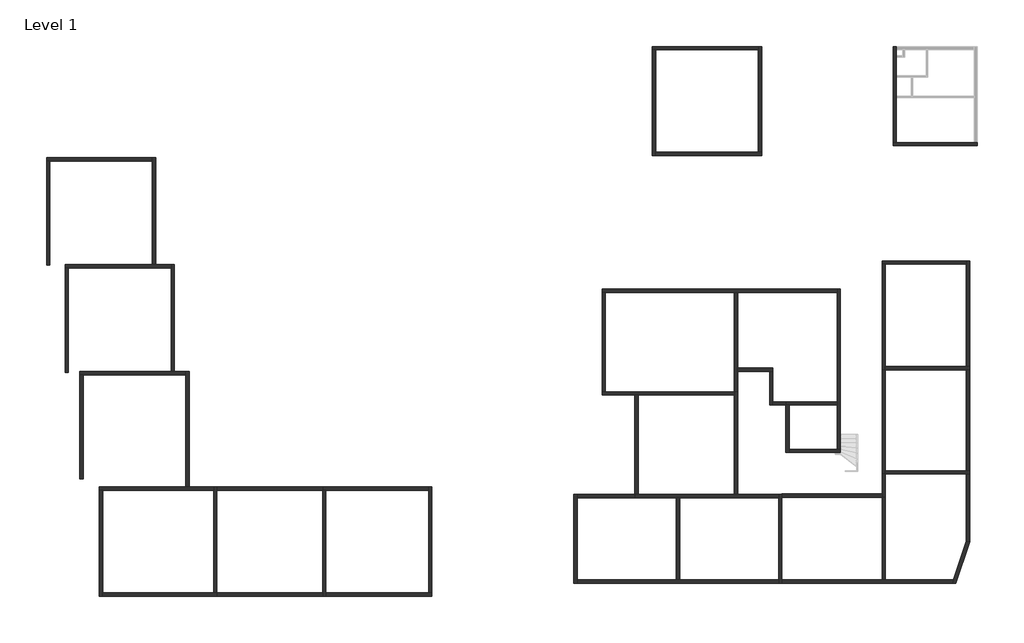
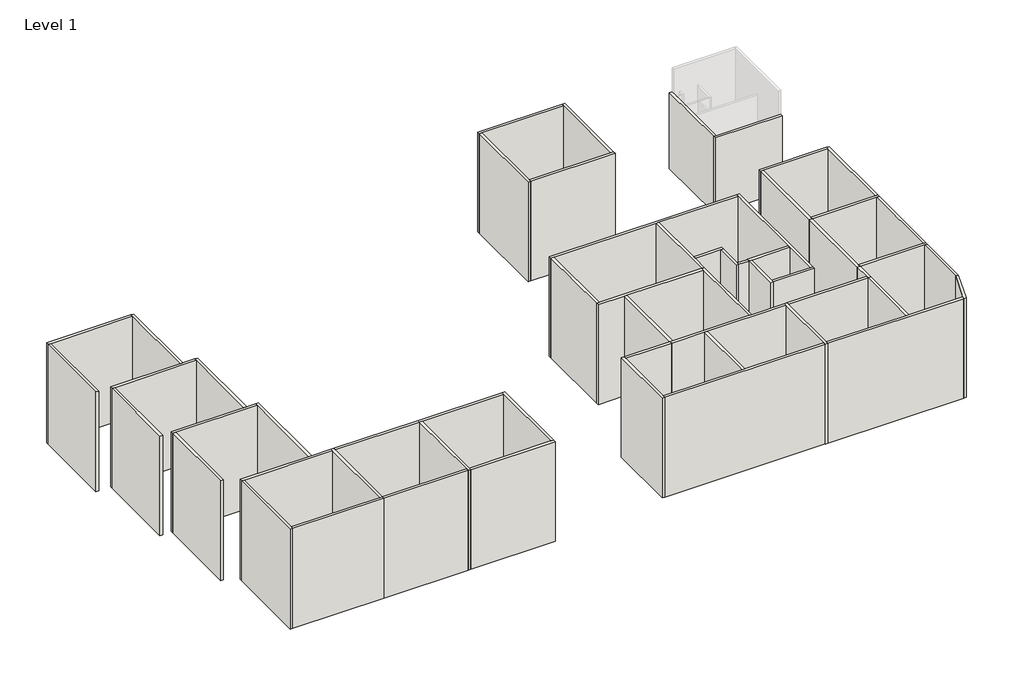
# One storey, part 1 of 2: 57 walls.
"""IFC4 building model written with IfcOpenShell, lengths in millimetres."""

from ifc_helpers import new_model, si_unit, origin, origin_with_axes, place, context, project, spatial, polyline, outline, extrude, faceted_brep, element, save

model = new_model("IFC4")

# Units and contexts
model_context = context("Model", 3, world=origin())
ifc_project = project(units=[si_unit("LENGTHUNIT", "METRE", prefix="MILLI")], contexts=[model_context])

# Site, building, storey
site = spatial("IfcSite", under=ifc_project)
building = spatial("IfcBuilding", under=site)
storey = spatial("IfcBuildingStorey", under=building, Name="Level 1", Elevation=0.0)

# Walls
placement = place(None, origin())
element("IfcWall", 1, ObjectType="Generic - 200mm", at=placement, inside=storey, context=model_context, shape_type="Brep", body=[
    faceted_brep([(30734.9948132, 14981.1915553, 0.0), (30534.9948132, 14981.1915553, 0.0), (25834.9948132, 14981.1915553, 0.0), (25634.9948132, 14981.1915553, 0.0), (25634.9948132, 14981.1915553, 6096.0), (25834.9948132, 14981.1915553, 6096.0), (30734.9948132, 14981.1915553, 6096.0), (30734.9948132, 14781.1915553, 0.0), (30734.9948132, 14781.1915553, 6096.0), (25634.9948132, 14781.1915553, 6096.0), (25634.9948132, 14781.1915553, 0.0)], [[[0, 1, 2, 3, 4, 5, 6]], [[7, 8, 9, 10]], [[3, 2, 1, 0, 7, 10]], [[6, 5, 4, 9, 8]], [[4, 3, 10, 9]], [[0, 6, 8, 7]]]),
])
element("IfcWall", 2, ObjectType="Generic - 200mm", at=placement, inside=storey, context=model_context, shape_type="Brep", body=[
    faceted_brep([(25834.9948132, 14981.1915553, 0.0), (25834.9948132, 17681.1915553, 0.0), (25834.9948132, 17781.1915553, 0.0), (25834.9948132, 18919.7859842, 0.0), (25834.9948132, 19019.7859842, 0.0), (25834.9948132, 20119.7859842, 0.0), (25834.9948132, 20219.7859842, 0.0), (25834.9948132, 20581.1915553, 0.0), (25834.9948132, 20781.1915553, 0.0), (25834.9948132, 20781.1915553, 6096.0), (25834.9948132, 20219.7859842, 6096.0), (25834.9948132, 20119.7859842, 6096.0), (25834.9948132, 19019.7859842, 6096.0), (25834.9948132, 18919.7859842, 6096.0), (25834.9948132, 17781.1915553, 6096.0), (25834.9948132, 17681.1915553, 6096.0), (25834.9948132, 14981.1915553, 6096.0), (25634.9948132, 14981.1915553, 0.0), (25634.9948132, 14981.1915553, 6096.0), (25634.9948132, 20781.1915553, 6096.0), (25634.9948132, 20781.1915553, 0.0)], [[[0, 1, 2, 3, 4, 5, 6, 7, 8, 9, 10, 11, 12, 13, 14, 15, 16]], [[17, 18, 19, 20]], [[8, 7, 6, 5, 4, 3, 2, 1, 0, 17, 20]], [[16, 15, 14, 13, 12, 11, 10, 9, 19, 18]], [[0, 16, 18, 17]], [[9, 8, 20, 19]]]),
])
element("IfcWall", 3, ObjectType="Generic - 200mm", at=placement, inside=storey, context=model_context, shape_type="Brep", body=[
    faceted_brep([(11094.267829, 20581.1915553, 0.0), (11294.267829, 20581.1915553, 0.0), (17494.267829, 20581.1915553, 0.0), (17494.267829, 20581.1915553, 8000.0), (11294.267829, 20581.1915553, 8000.0), (11094.267829, 20581.1915553, 8000.0), (11094.267829, 20781.1915553, 0.0), (11094.267829, 20781.1915553, 8000.0), (17494.267829, 20781.1915553, 8000.0), (17494.267829, 20781.1915553, 0.0)], [[[0, 1, 2, 3, 4, 5]], [[6, 7, 8, 9]], [[2, 1, 0, 6, 9]], [[5, 4, 3, 8, 7]], [[0, 5, 7, 6]], [[3, 2, 9, 8]]]),
])
element("IfcWall", 4, ObjectType="Generic - 200mm", at=placement, inside=storey, context=model_context, shape_type="Brep", body=[
    faceted_brep([(11294.267829, 14181.1915553, 0.0), (11294.267829, 14381.1915553, 0.0), (11294.267829, 20581.1915553, 0.0), (11294.267829, 20581.1915553, 8000.0), (11294.267829, 14381.1915553, 8000.0), (11294.267829, 14181.1915553, 8000.0), (11094.267829, 14181.1915553, 0.0), (11094.267829, 14181.1915553, 8000.0), (11094.267829, 20581.1915553, 8000.0), (11094.267829, 20581.1915553, 0.0)], [[[0, 1, 2, 3, 4, 5]], [[6, 7, 8, 9]], [[2, 1, 0, 6, 9]], [[5, 4, 3, 8, 7]], [[0, 5, 7, 6]], [[3, 2, 9, 8]]]),
])
element("IfcWall", 5, ObjectType="Generic - 200mm", at=placement, inside=storey, context=model_context, shape_type="Brep", body=[
    faceted_brep([(17694.267829, 14381.1915553, 0.0), (17494.267829, 14381.1915553, 0.0), (11294.267829, 14381.1915553, 0.0), (11294.267829, 14381.1915553, 8000.0), (17494.267829, 14381.1915553, 8000.0), (17694.267829, 14381.1915553, 8000.0), (17694.267829, 14181.1915553, 0.0), (17694.267829, 14181.1915553, 8000.0), (11294.267829, 14181.1915553, 8000.0), (11294.267829, 14181.1915553, 0.0)], [[[0, 1, 2, 3, 4, 5]], [[6, 7, 8, 9]], [[2, 1, 0, 6, 9]], [[5, 4, 3, 8, 7]], [[0, 5, 7, 6]], [[3, 2, 9, 8]]]),
])
element("IfcWall", 6, ObjectType="Generic - 200mm", at=placement, inside=storey, context=model_context, shape_type="Brep", body=[
    faceted_brep([(17494.267829, 20781.1915553, 0.0), (17494.267829, 20581.1915553, 0.0), (17494.267829, 14381.1915553, 0.0), (17494.267829, 14381.1915553, 8000.0), (17494.267829, 20581.1915553, 8000.0), (17494.267829, 20781.1915553, 8000.0), (17694.267829, 20781.1915553, 0.0), (17694.267829, 20781.1915553, 8000.0), (17694.267829, 14381.1915553, 8000.0), (17694.267829, 14381.1915553, 0.0)], [[[0, 1, 2, 3, 4, 5]], [[6, 7, 8, 9]], [[2, 1, 0, 6, 9]], [[5, 4, 3, 8, 7]], [[0, 5, 7, 6]], [[3, 2, 9, 8]]]),
])
element("IfcWall", 7, ObjectType="Generic - 200mm", at=placement, inside=storey, context=model_context, shape_type="Brep", body=[
    faceted_brep([(10039.836337, -6505.0098119, 0.0), (12539.836337, -6505.0098119, 0.0), (12739.836337, -6505.0098119, 0.0), (18719.836337, -6505.0098119, 0.0), (18719.836337, -6505.0098119, 8000.0), (12739.836337, -6505.0098119, 8000.0), (12539.836337, -6505.0098119, 8000.0), (10039.836337, -6505.0098119, 8000.0), (10039.836337, -6305.0098119, 0.0), (10039.836337, -6305.0098119, 8000.0), (10239.836337, -6305.0098119, 8000.0), (16039.836337, -6305.0098119, 8000.0), (16239.836337, -6305.0098119, 8000.0), (18719.836337, -6305.0098119, 8000.0), (18719.836337, -6305.0098119, 0.0), (16239.836337, -6305.0098119, 0.0), (16039.836337, -6305.0098119, 0.0), (10239.836337, -6305.0098119, 0.0)], [[[0, 1, 2, 3, 4, 5, 6, 7]], [[8, 9, 10, 11, 12, 13, 14, 15, 16, 17]], [[3, 2, 1, 0, 8, 17, 16, 15, 14]], [[7, 6, 5, 4, 13, 12, 11, 10, 9]], [[4, 3, 14, 13]], [[0, 7, 9, 8]]]),
])
element("IfcWall", 8, ObjectType="Generic - 200mm", at=placement, inside=storey, context=model_context, shape_type="Brep", body=[
    faceted_brep([(6549.836337, -11668.490171, 0.0), (6549.836337, -11468.490171, 0.0), (6549.836337, -6505.0098119, 0.0), (6549.836337, -6305.0098119, 0.0), (6549.836337, -6305.0098119, 8000.0), (6549.836337, -6505.0098119, 8000.0), (6549.836337, -11468.490171, 8000.0), (6549.836337, -11668.490171, 8000.0), (6349.836337, -11668.490171, 0.0), (6349.836337, -11668.490171, 8000.0), (6349.836337, -6305.0098119, 8000.0), (6349.836337, -6305.0098119, 0.0)], [[[0, 1, 2, 3, 4, 5, 6, 7]], [[8, 9, 10, 11]], [[3, 2, 1, 0, 8, 11]], [[7, 6, 5, 4, 10, 9]], [[0, 7, 9, 8]], [[4, 3, 11, 10]]]),
])
element("IfcWall", 9, ObjectType="Generic - 200mm", at=placement, inside=storey, context=model_context, shape_type="Brep", body=[
    faceted_brep([(18719.836337, -11468.490171, 0.0), (12739.836337, -11468.490171, 0.0), (12539.836337, -11468.490171, 0.0), (6549.836337, -11468.490171, 0.0), (6549.836337, -11468.490171, 8000.0), (12539.836337, -11468.490171, 8000.0), (12739.836337, -11468.490171, 8000.0), (18719.836337, -11468.490171, 8000.0), (18719.836337, -11668.490171, 0.0), (18719.836337, -11668.490171, 8000.0), (6549.836337, -11668.490171, 8000.0), (6549.836337, -11668.490171, 0.0)], [[[0, 1, 2, 3, 4, 5, 6, 7]], [[8, 9, 10, 11]], [[3, 2, 1, 0, 8, 11]], [[7, 6, 5, 4, 10, 9]], [[4, 3, 11, 10]], [[0, 7, 9, 8]]]),
])
element("IfcWall", 10, ObjectType="Generic - 200mm", at=placement, inside=storey, context=model_context, shape_type="Brep", body=[
    faceted_brep([(24968.3425199, 7619.475628, 0.0), (25168.3425199, 7619.475628, 0.0), (30068.3425199, 7619.475628, 0.0), (30068.3425199, 7619.475628, 8000.0), (25168.3425199, 7619.475628, 8000.0), (24968.3425199, 7619.475628, 8000.0), (24968.3425199, 7819.475628, 0.0), (24968.3425199, 7819.475628, 8000.0), (30068.3425199, 7819.475628, 8000.0), (30068.3425199, 7819.475628, 0.0)], [[[0, 1, 2, 3, 4, 5]], [[6, 7, 8, 9]], [[2, 1, 0, 6, 9]], [[5, 4, 3, 8, 7]], [[0, 5, 7, 6]], [[3, 2, 9, 8]]]),
])
element("IfcWall", 11, ObjectType="Generic - 200mm", at=placement, inside=storey, context=model_context, shape_type="Brep", body=[
    faceted_brep([(25168.3425199, 1219.475628, 0.0), (25168.3425199, 1419.475628, 0.0), (25168.3425199, 7619.475628, 0.0), (25168.3425199, 7619.475628, 8000.0), (25168.3425199, 1419.475628, 8000.0), (25168.3425199, 1219.475628, 8000.0), (24968.3425199, 1219.475628, 0.0), (24968.3425199, 1219.475628, 8000.0), (24968.3425199, 7619.475628, 8000.0), (24968.3425199, 7619.475628, 0.0), (24968.8612349, 1219.475628, 0.0), (24968.8612349, 1219.475628, 8000.0)], [[[0, 1, 2, 3, 4, 5]], [[6, 7, 8, 9]], [[2, 1, 0, 10, 6, 9]], [[5, 4, 3, 8, 7, 11]], [[0, 5, 11, 7, 6, 10]], [[3, 2, 9, 8]]]),
])
element("IfcWall", 12, ObjectType="Generic - 200mm", at=placement, inside=storey, context=model_context, shape_type="Brep", body=[
    faceted_brep([(30268.3425199, 1419.475628, 0.0), (30068.3425199, 1419.475628, 0.0), (25168.3425199, 1419.475628, 0.0), (25168.3425199, 1419.475628, 8000.0), (30068.3425199, 1419.475628, 8000.0), (30268.3425199, 1419.475628, 8000.0), (30268.3425199, 1219.475628, 0.0), (30268.3425199, 1219.475628, 8000.0), (30068.8612349, 1219.475628, 8000.0), (25168.8612349, 1219.475628, 8000.0), (25168.3425199, 1219.475628, 8000.0), (25168.3425199, 1219.475628, 0.0), (25168.8612349, 1219.475628, 0.0), (30068.8612349, 1219.475628, 0.0)], [[[0, 1, 2, 3, 4, 5]], [[6, 7, 8, 9, 10, 11, 12, 13]], [[2, 1, 0, 6, 13, 12, 11]], [[5, 4, 3, 10, 9, 8, 7]], [[0, 5, 7, 6]], [[3, 2, 11, 10]]]),
])
element("IfcWall", 13, ObjectType="Generic - 200mm", at=placement, inside=storey, context=model_context, shape_type="Brep", body=[
    faceted_brep([(30068.3425199, 7819.475628, 0.0), (30068.3425199, 7619.475628, 0.0), (30068.3425199, 1419.475628, 0.0), (30068.3425199, 1419.475628, 8000.0), (30068.3425199, 7619.475628, 8000.0), (30068.3425199, 7819.475628, 8000.0), (30268.3425199, 7819.475628, 0.0), (30268.3425199, 7819.475628, 8000.0), (30268.3425199, 1419.475628, 8000.0), (30268.3425199, 1419.475628, 0.0)], [[[0, 1, 2, 3, 4, 5]], [[6, 7, 8, 9]], [[2, 1, 0, 6, 9]], [[5, 4, 3, 8, 7]], [[0, 5, 7, 6]], [[3, 2, 9, 8]]]),
])
element("IfcWall", 14, ObjectType="Generic - 200mm", at=placement, inside=storey, context=model_context, shape_type="Brep", body=[
    faceted_brep([(25168.8612349, -5076.2808257, 0.0), (25168.8612349, -4876.2808257, 0.0), (25168.8612349, 1219.475628, 0.0), (25168.8612349, 1219.475628, 8000.0), (25168.8612349, -4876.2808257, 8000.0), (25168.8612349, -5076.2808257, 8000.0), (24968.8612349, -5076.2808257, 0.0), (24968.8612349, -5076.2808257, 8000.0), (24968.8612349, 1219.475628, 8000.0), (24968.8612349, 1219.475628, 0.0), (25168.3425199, 1219.475628, 0.0), (25168.3425199, 1219.475628, 8000.0)], [[[0, 1, 2, 3, 4, 5]], [[6, 7, 8, 9]], [[2, 1, 0, 6, 9, 10]], [[5, 4, 3, 11, 8, 7]], [[0, 5, 7, 6]], [[3, 2, 10, 9, 8, 11]]]),
])
element("IfcWall", 15, ObjectType="Generic - 200mm", at=placement, inside=storey, context=model_context, shape_type="Brep", body=[
    faceted_brep([(30268.8612349, -4876.2808257, 0.0), (30068.8612349, -4876.2808257, 0.0), (25168.8612349, -4876.2808257, 0.0), (25168.8612349, -4876.2808257, 8000.0), (30068.8612349, -4876.2808257, 8000.0), (30268.8612349, -4876.2808257, 8000.0), (30268.8612349, -5076.2808257, 0.0), (30268.8612349, -5076.2808257, 8000.0), (30069.3799498, -5076.2808257, 8000.0), (25168.8612349, -5076.2808257, 8000.0), (25168.8612349, -5076.2808257, 0.0), (30069.3799498, -5076.2808257, 0.0)], [[[0, 1, 2, 3, 4, 5]], [[6, 7, 8, 9, 10, 11]], [[2, 1, 0, 6, 11, 10]], [[5, 4, 3, 9, 8, 7]], [[0, 5, 7, 6]], [[3, 2, 10, 9]]]),
])
element("IfcWall", 16, ObjectType="Generic - 200mm", at=placement, inside=storey, context=model_context, shape_type="Brep", body=[
    faceted_brep([(30068.8612349, 1219.475628, 0.0), (30068.8612349, -4876.2808257, 0.0), (30068.8612349, -4876.2808257, 8000.0), (30068.8612349, 1219.475628, 8000.0), (30268.8612349, 1219.475628, 0.0), (30268.8612349, 1219.475628, 8000.0), (30268.8612349, -4876.2808257, 8000.0), (30268.8612349, -4876.2808257, 0.0), (30268.3425199, 1219.475628, 0.0), (30268.3425199, 1219.475628, 8000.0)], [[[0, 1, 2, 3]], [[4, 5, 6, 7]], [[1, 0, 8, 4, 7]], [[3, 2, 6, 5, 9]], [[2, 1, 7, 6]], [[0, 3, 9, 5, 4, 8]]]),
])
element("IfcWall", 17, ObjectType="Generic - 200mm", at=placement, inside=storey, context=model_context, shape_type="Brep", body=[
    faceted_brep([(30069.3799498, -5076.2808257, 0.0), (30069.3799498, -9143.0251929, 0.0), (30069.3799498, -9143.0251929, 8000.0), (30069.3799498, -5076.2808257, 8000.0), (30269.3799498, -5076.2808257, 0.0), (30269.3799498, -5076.2808257, 8000.0), (30269.3799498, -9175.863443, 8000.0), (30269.3799498, -9175.863443, 0.0), (30268.8612349, -5076.2808257, 0.0), (30268.8612349, -5076.2808257, 8000.0)], [[[0, 1, 2, 3]], [[4, 5, 6, 7]], [[1, 0, 8, 4, 7]], [[3, 2, 6, 5, 9]], [[0, 3, 9, 5, 4, 8]], [[2, 1, 7, 6]]]),
])
element("IfcWall", 18, ObjectType="Generic - 200mm", at=placement, inside=storey, context=model_context, shape_type="Brep", body=[
    faceted_brep([(19150.6041014, -900.524372, 0.0), (19350.6041014, -900.524372, 0.0), (22249.836337, -900.524372, 0.0), (22249.836337, -900.524372, 8000.0), (19350.6041014, -900.524372, 8000.0), (19150.6041014, -900.524372, 8000.0), (19150.6041014, -700.524372, 0.0), (19150.6041014, -700.524372, 8000.0), (22249.836337, -700.524372, 8000.0), (22249.836337, -700.524372, 0.0)], [[[0, 1, 2, 3, 4, 5]], [[6, 7, 8, 9]], [[2, 1, 0, 6, 9]], [[5, 4, 3, 8, 7]], [[0, 5, 7, 6]], [[3, 2, 9, 8]]]),
])
element("IfcWall", 19, ObjectType="Generic - 200mm", at=placement, inside=storey, context=model_context, shape_type="Brep", body=[
    faceted_brep([(19350.6041014, -3776.2808257, 0.0), (19350.6041014, -3576.2808257, 0.0), (19350.6041014, -900.524372, 0.0), (19350.6041014, -900.524372, 8000.0), (19350.6041014, -3576.2808257, 8000.0), (19350.6041014, -3776.2808257, 8000.0), (19150.6041014, -3776.2808257, 0.0), (19150.6041014, -3776.2808257, 8000.0), (19150.6041014, -900.524372, 8000.0), (19150.6041014, -900.524372, 0.0)], [[[0, 1, 2, 3, 4, 5]], [[6, 7, 8, 9]], [[2, 1, 0, 6, 9]], [[5, 4, 3, 8, 7]], [[0, 5, 7, 6]], [[3, 2, 9, 8]]]),
])
element("IfcWall", 20, ObjectType="Generic - 200mm", at=placement, inside=storey, context=model_context, shape_type="Brep", body=[
    faceted_brep([(22449.836337, -3576.2808257, 0.0), (22249.836337, -3576.2808257, 0.0), (19350.6041014, -3576.2808257, 0.0), (19350.6041014, -3576.2808257, 8000.0), (22249.836337, -3576.2808257, 8000.0), (22449.836337, -3576.2808257, 8000.0), (22449.836337, -3776.2808257, 0.0), (22449.836337, -3776.2808257, 8000.0), (19350.6041014, -3776.2808257, 8000.0), (19350.6041014, -3776.2808257, 0.0)], [[[0, 1, 2, 3, 4, 5]], [[6, 7, 8, 9]], [[2, 1, 0, 6, 9]], [[5, 4, 3, 8, 7]], [[3, 2, 9, 8]], [[0, 5, 7, 6]]]),
])
element("IfcWall", 21, ObjectType="Generic - 200mm", at=placement, inside=storey, context=model_context, shape_type="Brep", body=[
    faceted_brep([(18919.836337, -11676.6907835, 0.0), (18919.836337, -11476.6907835, 0.0), (18919.836337, -6476.2808257, 0.0), (18919.836337, -6305.0098119, 0.0), (18919.836337, -6305.0098119, 8000.0), (18919.836337, -6476.2808257, 8000.0), (18919.836337, -11476.6907835, 8000.0), (18919.836337, -11676.6907835, 8000.0), (18719.836337, -11676.6907835, 0.0), (18719.836337, -11676.6907835, 8000.0), (18719.836337, -11668.490171, 8000.0), (18719.836337, -11468.490171, 8000.0), (18719.836337, -6505.0098119, 8000.0), (18719.836337, -6305.0098119, 8000.0), (18719.836337, -6305.0098119, 0.0), (18719.836337, -6505.0098119, 0.0), (18719.836337, -11468.490171, 0.0), (18719.836337, -11668.490171, 0.0)], [[[0, 1, 2, 3, 4, 5, 6, 7]], [[8, 9, 10, 11, 12, 13, 14, 15, 16, 17]], [[3, 2, 1, 0, 8, 17, 16, 15, 14]], [[7, 6, 5, 4, 13, 12, 11, 10, 9]], [[0, 7, 9, 8]], [[4, 3, 14, 13]]]),
])
element("IfcWall", 22, ObjectType="Generic - 200mm", at=placement, inside=storey, context=model_context, shape_type="Brep", body=[
    faceted_brep([(29281.8131798, -11476.6907835, 0.0), (25168.8612349, -11476.6907835, 0.0), (24968.8612349, -11476.6907835, 0.0), (18919.836337, -11476.6907835, 0.0), (18919.836337, -11476.6907835, 8000.0), (24968.8612349, -11476.6907835, 8000.0), (25168.8612349, -11476.6907835, 8000.0), (29281.8131798, -11476.6907835, 8000.0), (29214.3170678, -11676.6907835, 0.0), (29214.3170678, -11676.6907835, 8000.0), (18919.836337, -11676.6907835, 8000.0), (18919.836337, -11676.6907835, 0.0)], [[[0, 1, 2, 3, 4, 5, 6, 7]], [[8, 9, 10, 11]], [[3, 2, 1, 0, 8, 11]], [[7, 6, 5, 4, 10, 9]], [[4, 3, 11, 10]], [[0, 7, 9, 8]]]),
])
element("IfcWall", 23, ObjectType="Generic - 200mm", at=placement, inside=storey, context=model_context, shape_type="Brep", body=[
    faceted_brep([(22449.836337, -3576.2808257, 0.0), (22449.836337, 6101.390757, 0.0), (22449.836337, 6101.390757, 8000.0), (22449.836337, -3576.2808257, 8000.0), (22249.836337, -3576.2808257, 0.0), (22249.836337, -3576.2808257, 8000.0), (22249.836337, -900.524372, 8000.0), (22249.836337, -700.524372, 8000.0), (22249.836337, 5901.390757, 8000.0), (22249.836337, 6101.390757, 8000.0), (22249.836337, 6101.390757, 0.0), (22249.836337, 5901.390757, 0.0), (22249.836337, -700.524372, 0.0), (22249.836337, -900.524372, 0.0)], [[[0, 1, 2, 3]], [[4, 5, 6, 7, 8, 9, 10, 11, 12, 13]], [[1, 0, 4, 13, 12, 11, 10]], [[3, 2, 9, 8, 7, 6, 5]], [[0, 3, 5, 4]], [[2, 1, 10, 9]]]),
])
element("IfcWall", 24, ObjectType="Generic - 200mm", at=placement, inside=storey, context=model_context, shape_type="Brep", body=[
    faceted_brep([(-2430.0032836, -5850.5375199, 0.0), (-2430.0032836, -6050.5375199, 0.0), (-2430.0032836, -12250.5375199, 0.0), (-2430.0032836, -12250.5375199, 8000.0), (-2430.0032836, -6050.5375199, 8000.0), (-2430.0032836, -5850.5375199, 8000.0), (-2230.0032836, -5850.5375199, 0.0), (-2230.0032836, -5850.5375199, 8000.0), (-2230.0032836, -12250.5375199, 8000.0), (-2230.0032836, -12250.5375199, 0.0)], [[[0, 1, 2, 3, 4, 5]], [[6, 7, 8, 9]], [[2, 1, 0, 6, 9]], [[5, 4, 3, 8, 7]], [[0, 5, 7, 6]], [[3, 2, 9, 8]]]),
])
element("IfcWall", 25, ObjectType="Generic - 200mm", at=placement, inside=storey, context=model_context, shape_type="Brep", body=[
    faceted_brep([(-8830.0032836, -6050.5375199, 0.0), (-8630.0032836, -6050.5375199, 0.0), (-2430.0032836, -6050.5375199, 0.0), (-2430.0032836, -6050.5375199, 8000.0), (-8630.0032836, -6050.5375199, 8000.0), (-8830.0032836, -6050.5375199, 8000.0), (-8830.0032836, -5850.5375199, 0.0), (-8830.0032836, -5850.5375199, 8000.0), (-2430.0032836, -5850.5375199, 8000.0), (-2430.0032836, -5850.5375199, 0.0), (-8830.0032836, -5851.0562349, 0.0), (-8830.0032836, -5851.0562349, 8000.0)], [[[0, 1, 2, 3, 4, 5]], [[6, 7, 8, 9]], [[2, 1, 0, 10, 6, 9]], [[5, 4, 3, 8, 7, 11]], [[0, 5, 11, 7, 6, 10]], [[3, 2, 9, 8]]]),
])
element("IfcWall", 26, ObjectType="Generic - 200mm", at=placement, inside=storey, context=model_context, shape_type="Brep", body=[
    faceted_brep([(-8630.0032836, -12450.5375199, 0.0), (-8630.0032836, -12250.5375199, 0.0), (-8630.0032836, -6050.5375199, 0.0), (-8630.0032836, -6050.5375199, 8000.0), (-8630.0032836, -12250.5375199, 8000.0), (-8630.0032836, -12450.5375199, 8000.0), (-8830.0032836, -12450.5375199, 0.0), (-8830.0032836, -12450.5375199, 8000.0), (-8830.0032836, -12251.0562349, 8000.0), (-8830.0032836, -6051.0562349, 8000.0), (-8830.0032836, -6050.5375199, 8000.0), (-8830.0032836, -6050.5375199, 0.0), (-8830.0032836, -6051.0562349, 0.0), (-8830.0032836, -12251.0562349, 0.0)], [[[0, 1, 2, 3, 4, 5]], [[6, 7, 8, 9, 10, 11, 12, 13]], [[2, 1, 0, 6, 13, 12, 11]], [[5, 4, 3, 10, 9, 8, 7]], [[0, 5, 7, 6]], [[3, 2, 11, 10]]]),
])
element("IfcWall", 27, ObjectType="Generic - 200mm", at=placement, inside=storey, context=model_context, shape_type="Brep", body=[
    faceted_brep([(-2230.0032836, -12250.5375199, 0.0), (-2430.0032836, -12250.5375199, 0.0), (-8630.0032836, -12250.5375199, 0.0), (-8630.0032836, -12250.5375199, 8000.0), (-2430.0032836, -12250.5375199, 8000.0), (-2230.0032836, -12250.5375199, 8000.0), (-2230.0032836, -12450.5375199, 0.0), (-2230.0032836, -12450.5375199, 8000.0), (-8630.0032836, -12450.5375199, 8000.0), (-8630.0032836, -12450.5375199, 0.0)], [[[0, 1, 2, 3, 4, 5]], [[6, 7, 8, 9]], [[2, 1, 0, 6, 9]], [[5, 4, 3, 8, 7]], [[0, 5, 7, 6]], [[3, 2, 9, 8]]]),
])
element("IfcWall", 28, ObjectType="Generic - 200mm", at=placement, inside=storey, context=model_context, shape_type="Brep", body=[
    faceted_brep([(-15225.7597372, -6051.0562349, 0.0), (-8830.0032836, -6051.0562349, 0.0), (-8830.0032836, -6051.0562349, 8000.0), (-15225.7597372, -6051.0562349, 8000.0), (-15225.7597372, -5851.0562349, 0.0), (-15225.7597372, -5851.0562349, 8000.0), (-8830.0032836, -5851.0562349, 8000.0), (-8830.0032836, -5851.0562349, 0.0), (-8830.0032836, -6050.5375199, 0.0), (-8830.0032836, -6050.5375199, 8000.0)], [[[0, 1, 2, 3]], [[4, 5, 6, 7]], [[1, 0, 4, 7, 8]], [[3, 2, 9, 6, 5]], [[2, 1, 8, 7, 6, 9]], [[0, 3, 5, 4]]]),
])
element("IfcWall", 29, ObjectType="Generic - 200mm", at=placement, inside=storey, context=model_context, shape_type="Brep", body=[
    faceted_brep([(-8830.0032836, -12251.0562349, 0.0), (-15225.7597372, -12251.0562349, 0.0), (-15225.7597372, -12251.0562349, 8000.0), (-8830.0032836, -12251.0562349, 8000.0), (-8830.0032836, -12451.0562349, 0.0), (-8830.0032836, -12451.0562349, 8000.0), (-15225.7597372, -12451.0562349, 8000.0), (-15225.7597372, -12451.0562349, 0.0), (-8830.0032836, -12450.5375199, 0.0), (-8830.0032836, -12450.5375199, 8000.0)], [[[0, 1, 2, 3]], [[4, 5, 6, 7]], [[1, 0, 8, 4, 7]], [[3, 2, 6, 5, 9]], [[0, 3, 9, 5, 4, 8]], [[2, 1, 7, 6]]]),
])
element("IfcWall", 30, ObjectType="Generic - 200mm", at=placement, inside=storey, context=model_context, shape_type="Brep", body=[
    faceted_brep([(-25515.2414934, 13854.6128579, 0.0), (-25315.2414934, 13854.6128579, 0.0), (-19115.2414934, 13854.6128579, 0.0), (-19115.2414934, 13854.6128579, 8000.0), (-25315.2414934, 13854.6128579, 8000.0), (-25515.2414934, 13854.6128579, 8000.0), (-25515.2414934, 14054.6128579, 0.0), (-25515.2414934, 14054.6128579, 8000.0), (-19115.2414934, 14054.6128579, 8000.0), (-19115.2414934, 14054.6128579, 0.0)], [[[0, 1, 2, 3, 4, 5]], [[6, 7, 8, 9]], [[2, 1, 0, 6, 9]], [[5, 4, 3, 8, 7]], [[0, 5, 7, 6]], [[3, 2, 9, 8]]]),
])
element("IfcWall", 31, ObjectType="Generic - 200mm", at=placement, inside=storey, context=model_context, shape_type="SweptSolid", body=[
    extrude(outline(polyline([(-25315.2414934, 13854.6128579), (-25315.2414934, 7554.6128579), (-25515.2414934, 7554.6128579), (-25515.2414934, 13854.6128579), (-25315.2414934, 13854.6128579)])), origin_with_axes(), (0.0, 0.0, 1.0), 8000.0),
])
element("IfcWall", 32, ObjectType="Generic - 200mm", at=placement, inside=storey, context=model_context, shape_type="Brep", body=[
    faceted_brep([(-19115.2414934, 14054.6128579, 0.0), (-19115.2414934, 13854.6128579, 0.0), (-19115.2414934, 7585.232767, 0.0), (-19115.2414934, 7585.232767, 8000.0), (-19115.2414934, 13854.6128579, 8000.0), (-19115.2414934, 14054.6128579, 8000.0), (-18915.2414934, 14054.6128579, 0.0), (-18915.2414934, 14054.6128579, 8000.0), (-18915.2414934, 7585.232767, 8000.0), (-18915.2414934, 7585.232767, 0.0)], [[[0, 1, 2, 3, 4, 5]], [[6, 7, 8, 9]], [[2, 1, 0, 6, 9]], [[5, 4, 3, 8, 7]], [[0, 5, 7, 6]], [[3, 2, 9, 8]]]),
])
element("IfcWall", 33, ObjectType="Generic - 200mm", at=placement, inside=storey, context=model_context, shape_type="Brep", body=[
    faceted_brep([(-24394.8529907, 7385.232767, 0.0), (-24194.8529907, 7385.232767, 0.0), (-17994.8529907, 7385.232767, 0.0), (-17994.8529907, 7385.232767, 8000.0), (-24194.8529907, 7385.232767, 8000.0), (-24394.8529907, 7385.232767, 8000.0), (-24394.8529907, 7585.232767, 0.0), (-24394.8529907, 7585.232767, 8000.0), (-19115.2414934, 7585.232767, 8000.0), (-18915.2414934, 7585.232767, 8000.0), (-17994.8529907, 7585.232767, 8000.0), (-17994.8529907, 7585.232767, 0.0), (-18915.2414934, 7585.232767, 0.0), (-19115.2414934, 7585.232767, 0.0)], [[[0, 1, 2, 3, 4, 5]], [[6, 7, 8, 9, 10, 11, 12, 13]], [[2, 1, 0, 6, 13, 12, 11]], [[5, 4, 3, 10, 9, 8, 7]], [[0, 5, 7, 6]], [[3, 2, 11, 10]]]),
])
element("IfcWall", 34, ObjectType="Generic - 200mm", at=placement, inside=storey, context=model_context, shape_type="SweptSolid", body=[
    extrude(outline(polyline([(-24194.8529907, 7385.232767), (-24194.8529907, 1085.232767), (-24394.8529907, 1085.232767), (-24394.8529907, 7385.232767), (-24194.8529907, 7385.232767)])), origin_with_axes(), (0.0, 0.0, 1.0), 8000.0),
])
element("IfcWall", 35, ObjectType="Generic - 200mm", at=placement, inside=storey, context=model_context, shape_type="Brep", body=[
    faceted_brep([(-17994.8529907, 7585.232767, 0.0), (-17994.8529907, 7385.232767, 0.0), (-17994.8529907, 1134.2648187, 0.0), (-17994.8529907, 1134.2648187, 8000.0), (-17994.8529907, 7385.232767, 8000.0), (-17994.8529907, 7585.232767, 8000.0), (-17794.8529907, 7585.232767, 0.0), (-17794.8529907, 7585.232767, 8000.0), (-17794.8529907, 1134.2648187, 8000.0), (-17794.8529907, 1134.2648187, 0.0)], [[[0, 1, 2, 3, 4, 5]], [[6, 7, 8, 9]], [[2, 1, 0, 6, 9]], [[5, 4, 3, 8, 7]], [[0, 5, 7, 6]], [[3, 2, 9, 8]]]),
])
element("IfcWall", 36, ObjectType="Generic - 200mm", at=placement, inside=storey, context=model_context, shape_type="Brep", body=[
    faceted_brep([(-23499.9022694, 934.2648187, 0.0), (-23299.9022694, 934.2648187, 0.0), (-17099.9022694, 934.2648187, 0.0), (-17099.9022694, 934.2648187, 8000.0), (-23299.9022694, 934.2648187, 8000.0), (-23499.9022694, 934.2648187, 8000.0), (-23499.9022694, 1134.2648187, 0.0), (-23499.9022694, 1134.2648187, 8000.0), (-17994.8529907, 1134.2648187, 8000.0), (-17794.8529907, 1134.2648187, 8000.0), (-17099.9022694, 1134.2648187, 8000.0), (-17099.9022694, 1134.2648187, 0.0), (-17794.8529907, 1134.2648187, 0.0), (-17994.8529907, 1134.2648187, 0.0)], [[[0, 1, 2, 3, 4, 5]], [[6, 7, 8, 9, 10, 11, 12, 13]], [[2, 1, 0, 6, 13, 12, 11]], [[5, 4, 3, 10, 9, 8, 7]], [[0, 5, 7, 6]], [[3, 2, 11, 10]]]),
])
element("IfcWall", 37, ObjectType="Generic - 200mm", at=placement, inside=storey, context=model_context, shape_type="SweptSolid", body=[
    extrude(outline(polyline([(-23299.9022694, 934.2648187), (-23299.9022694, -5365.7351813), (-23499.9022694, -5365.7351813), (-23499.9022694, 934.2648187), (-23299.9022694, 934.2648187)])), origin_with_axes(), (0.0, 0.0, 1.0), 8000.0),
])
element("IfcWall", 38, ObjectType="Generic - 200mm", at=placement, inside=storey, context=model_context, shape_type="Brep", body=[
    faceted_brep([(-17099.9022694, 1134.2648187, 0.0), (-17099.9022694, 934.2648187, 0.0), (-17099.9022694, -5851.0562349, 0.0), (-17099.9022694, -5851.0562349, 8000.0), (-17099.9022694, 934.2648187, 8000.0), (-17099.9022694, 1134.2648187, 8000.0), (-16899.9022694, 1134.2648187, 0.0), (-16899.9022694, 1134.2648187, 8000.0), (-16899.9022694, -5851.0562349, 8000.0), (-16899.9022694, -5851.0562349, 0.0)], [[[0, 1, 2, 3, 4, 5]], [[6, 7, 8, 9]], [[2, 1, 0, 6, 9]], [[5, 4, 3, 8, 7]], [[0, 5, 7, 6]], [[3, 2, 9, 8]]]),
])
element("IfcWall", 39, ObjectType="Generic - 200mm", at=placement, inside=storey, context=model_context, shape_type="Brep", body=[
    faceted_brep([(-22325.7597372, -6051.0562349, 0.0), (-22125.7597372, -6051.0562349, 0.0), (-15425.7597372, -6051.0562349, 0.0), (-15425.7597372, -6051.0562349, 8000.0), (-22125.7597372, -6051.0562349, 8000.0), (-22325.7597372, -6051.0562349, 8000.0), (-22325.7597372, -5851.0562349, 0.0), (-22325.7597372, -5851.0562349, 8000.0), (-17099.9022694, -5851.0562349, 8000.0), (-16899.9022694, -5851.0562349, 8000.0), (-15425.7597372, -5851.0562349, 8000.0), (-15425.7597372, -5851.0562349, 0.0), (-16899.9022694, -5851.0562349, 0.0), (-17099.9022694, -5851.0562349, 0.0)], [[[0, 1, 2, 3, 4, 5]], [[6, 7, 8, 9, 10, 11, 12, 13]], [[2, 1, 0, 6, 13, 12, 11]], [[5, 4, 3, 10, 9, 8, 7]], [[0, 5, 7, 6]], [[3, 2, 11, 10]]]),
])
element("IfcWall", 40, ObjectType="Generic - 200mm", at=placement, inside=storey, context=model_context, shape_type="Brep", body=[
    faceted_brep([(-22125.7597372, -12451.0562349, 0.0), (-22125.7597372, -12251.0562349, 0.0), (-22125.7597372, -6051.0562349, 0.0), (-22125.7597372, -6051.0562349, 8000.0), (-22125.7597372, -12251.0562349, 8000.0), (-22125.7597372, -12451.0562349, 8000.0), (-22325.7597372, -12451.0562349, 0.0), (-22325.7597372, -12451.0562349, 8000.0), (-22325.7597372, -6051.0562349, 8000.0), (-22325.7597372, -6051.0562349, 0.0)], [[[0, 1, 2, 3, 4, 5]], [[6, 7, 8, 9]], [[2, 1, 0, 6, 9]], [[5, 4, 3, 8, 7]], [[0, 5, 7, 6]], [[3, 2, 9, 8]]]),
])
element("IfcWall", 41, ObjectType="Generic - 200mm", at=placement, inside=storey, context=model_context, shape_type="Brep", body=[
    faceted_brep([(-15225.7597372, -12251.0562349, 0.0), (-15425.7597372, -12251.0562349, 0.0), (-22125.7597372, -12251.0562349, 0.0), (-22125.7597372, -12251.0562349, 8000.0), (-15425.7597372, -12251.0562349, 8000.0), (-15225.7597372, -12251.0562349, 8000.0), (-15225.7597372, -12451.0562349, 0.0), (-15225.7597372, -12451.0562349, 8000.0), (-22125.7597372, -12451.0562349, 8000.0), (-22125.7597372, -12451.0562349, 0.0)], [[[0, 1, 2, 3, 4, 5]], [[6, 7, 8, 9]], [[2, 1, 0, 6, 9]], [[5, 4, 3, 8, 7]], [[0, 5, 7, 6]], [[3, 2, 9, 8]]]),
])
element("IfcWall", 42, ObjectType="Generic - 200mm", at=placement, inside=storey, context=model_context, shape_type="Brep", body=[
    faceted_brep([(-15425.7597372, -5851.0562349, 0.0), (-15425.7597372, -6051.0562349, 0.0), (-15425.7597372, -12251.0562349, 0.0), (-15425.7597372, -12251.0562349, 8000.0), (-15425.7597372, -6051.0562349, 8000.0), (-15425.7597372, -5851.0562349, 8000.0), (-15225.7597372, -5851.0562349, 0.0), (-15225.7597372, -5851.0562349, 8000.0), (-15225.7597372, -6051.0562349, 8000.0), (-15225.7597372, -12251.0562349, 8000.0), (-15225.7597372, -12251.0562349, 0.0), (-15225.7597372, -6051.0562349, 0.0)], [[[0, 1, 2, 3, 4, 5]], [[6, 7, 8, 9, 10, 11]], [[2, 1, 0, 6, 11, 10]], [[5, 4, 3, 9, 8, 7]], [[0, 5, 7, 6]], [[3, 2, 10, 9]]]),
])
element("IfcWall", 43, ObjectType="Generic - 200mm", at=placement, inside=storey, context=model_context, shape_type="Brep", body=[
    faceted_brep([(16039.836337, -98.609243, 0.0), (16039.836337, -298.609243, 0.0), (16039.836337, -6305.0098119, 0.0), (16039.836337, -6305.0098119, 8000.0), (16039.836337, -298.609243, 8000.0), (16039.836337, -98.609243, 8000.0), (16239.836337, -98.609243, 0.0), (16239.836337, -98.609243, 8000.0), (16239.836337, -6305.0098119, 8000.0), (16239.836337, -6305.0098119, 0.0)], [[[0, 1, 2, 3, 4, 5]], [[6, 7, 8, 9]], [[2, 1, 0, 6, 9]], [[5, 4, 3, 8, 7]], [[3, 2, 9, 8]], [[0, 5, 7, 6]]]),
])
element("IfcWall", 44, ObjectType="Generic - 200mm", at=placement, inside=storey, context=model_context, shape_type="Brep", body=[
    faceted_brep([(8048.9259597, -298.609243, 0.0), (10039.836337, -298.609243, 0.0), (10239.836337, -298.609243, 0.0), (16039.836337, -298.609243, 0.0), (16039.836337, -298.609243, 8000.0), (10239.836337, -298.609243, 8000.0), (10039.836337, -298.609243, 8000.0), (8048.9259597, -298.609243, 8000.0), (8048.9259597, -98.609243, 0.0), (8048.9259597, -98.609243, 8000.0), (8248.9259597, -98.609243, 8000.0), (16039.836337, -98.609243, 8000.0), (16039.836337, -98.609243, 0.0), (8248.9259597, -98.609243, 0.0)], [[[0, 1, 2, 3, 4, 5, 6, 7]], [[8, 9, 10, 11, 12, 13]], [[3, 2, 1, 0, 8, 13, 12]], [[7, 6, 5, 4, 11, 10, 9]], [[4, 3, 12, 11]], [[0, 7, 9, 8]]]),
])
element("IfcWall", 45, ObjectType="Generic - 200mm", at=placement, inside=storey, context=model_context, shape_type="Brep", body=[
    faceted_brep([(8048.9259597, 5901.390757, 0.0), (8248.9259597, 5901.390757, 0.0), (16039.836337, 5901.390757, 0.0), (16239.836337, 5901.390757, 0.0), (22249.836337, 5901.390757, 0.0), (22249.836337, 5901.390757, 8000.0), (16239.836337, 5901.390757, 8000.0), (16039.836337, 5901.390757, 8000.0), (8248.9259597, 5901.390757, 8000.0), (8048.9259597, 5901.390757, 8000.0), (8048.9259597, 6101.390757, 0.0), (8048.9259597, 6101.390757, 8000.0), (22249.836337, 6101.390757, 8000.0), (22249.836337, 6101.390757, 0.0)], [[[0, 1, 2, 3, 4, 5, 6, 7, 8, 9]], [[10, 11, 12, 13]], [[4, 3, 2, 1, 0, 10, 13]], [[9, 8, 7, 6, 5, 12, 11]], [[5, 4, 13, 12]], [[0, 9, 11, 10]]]),
])
element("IfcWall", 46, ObjectType="Generic - 200mm", at=placement, inside=storey, context=model_context, shape_type="SweptSolid", body=[
    extrude(outline(polyline([(24968.8612349, -11476.6907835), (24968.8612349, -6476.2808257), (25168.8612349, -6476.2808257), (25168.8612349, -11476.6907835), (24968.8612349, -11476.6907835)])), origin_with_axes(), (0.0, 0.0, 1.0), 8000.0),
])
element("IfcWall", 47, ObjectType="Generic - 200mm", at=placement, inside=storey, context=model_context, shape_type="Brep", body=[
    faceted_brep([(30069.3799498, -9143.0251929, 0.0), (29281.8131798, -11476.6907835, 0.0), (29214.3170678, -11676.6907835, 0.0), (29214.3170678, -11676.6907835, 8000.0), (29281.8131798, -11476.6907835, 8000.0), (30069.3799498, -9143.0251929, 8000.0), (30269.3799498, -9175.863443, 0.0), (30269.3799498, -9175.863443, 8000.0), (29425.3993388, -11676.6907835, 8000.0), (29425.3993388, -11676.6907835, 0.0)], [[[0, 1, 2, 3, 4, 5]], [[6, 7, 8, 9]], [[2, 1, 0, 6, 9]], [[5, 4, 3, 8, 7]], [[0, 5, 7, 6]], [[3, 2, 9, 8]]]),
])
element("IfcWall", 48, ObjectType="Generic - 200mm", at=placement, inside=storey, context=model_context, shape_type="Brep", body=[
    faceted_brep([(24968.8612349, -5076.2808257, 0.0), (24968.8612349, -6276.2808257, 0.0), (24968.8612349, -6476.2808257, 0.0), (24968.8612349, -6476.2808257, 8000.0), (24968.8612349, -6276.2808257, 8000.0), (24968.8612349, -5076.2808257, 8000.0), (25168.8612349, -5076.2808257, 0.0), (25168.8612349, -5076.2808257, 8000.0), (25168.8612349, -6476.2808257, 8000.0), (25168.8612349, -6476.2808257, 0.0)], [[[0, 1, 2, 3, 4, 5]], [[6, 7, 8, 9]], [[2, 1, 0, 6, 9]], [[5, 4, 3, 8, 7]], [[0, 5, 7, 6]], [[3, 2, 9, 8]]]),
])
element("IfcWall", 49, ObjectType="Generic - 200mm", at=placement, inside=storey, context=model_context, shape_type="Brep", body=[
    faceted_brep([(24968.8612349, -6276.2808257, 0.0), (18919.836337, -6276.2808257, 0.0), (18919.836337, -6276.2808257, 8000.0), (24968.8612349, -6276.2808257, 8000.0), (24968.8612349, -6476.2808257, 0.0), (24968.8612349, -6476.2808257, 8000.0), (18919.836337, -6476.2808257, 8000.0), (18919.836337, -6476.2808257, 0.0), (18919.836337, -6305.0098119, 0.0), (18919.836337, -6305.0098119, 8000.0)], [[[0, 1, 2, 3]], [[4, 5, 6, 7]], [[1, 0, 4, 7, 8]], [[3, 2, 9, 6, 5]], [[0, 3, 5, 4]], [[2, 1, 8, 7, 6, 9]]]),
])
element("IfcWall", 50, ObjectType="Generic - 200mm", at=placement, inside=storey, context=model_context, shape_type="SweptSolid", body=[
    extrude(outline(polyline([(12539.836337, -11468.490171), (12539.836337, -6505.0098119), (12739.836337, -6505.0098119), (12739.836337, -11468.490171), (12539.836337, -11468.490171)])), origin_with_axes(), (0.0, 0.0, 1.0), 8000.0),
])
element("IfcWall", 51, ObjectType="Generic - 200mm", at=placement, inside=storey, context=model_context, shape_type="SweptSolid", body=[
    extrude(outline(polyline([(10039.836337, -6305.0098119), (10039.836337, -298.609243), (10239.836337, -298.609243), (10239.836337, -6305.0098119), (10039.836337, -6305.0098119)])), origin_with_axes(), (0.0, 0.0, 1.0), 8000.0),
])
element("IfcWall", 52, ObjectType="Generic - 200mm", at=placement, inside=storey, context=model_context, shape_type="SweptSolid", body=[
    extrude(outline(polyline([(8048.9259597, -98.609243), (8048.9259597, 5901.390757), (8248.9259597, 5901.390757), (8248.9259597, -98.609243), (8048.9259597, -98.609243)])), origin_with_axes(), (0.0, 0.0, 1.0), 8000.0),
])
element("IfcWall", 53, ObjectType="Generic - 200mm", at=placement, inside=storey, context=model_context, shape_type="SweptSolid", body=[
    extrude(outline(polyline([(6549.836337, -6305.0098119), (10039.836337, -6305.0098119), (10039.836337, -6505.0098119), (6549.836337, -6505.0098119), (6549.836337, -6305.0098119)])), origin_with_axes(), (0.0, 0.0, 1.0), 8000.0),
])
element("IfcWall", 54, ObjectType="Generic - 200mm", at=placement, inside=storey, context=model_context, shape_type="Brep", body=[
    faceted_brep([(16239.836337, -98.609243, 0.0), (16239.836337, 1139.475628, 0.0), (16239.836337, 1339.475628, 0.0), (16239.836337, 5901.390757, 0.0), (16239.836337, 5901.390757, 8000.0), (16239.836337, 1339.475628, 8000.0), (16239.836337, 1139.475628, 8000.0), (16239.836337, -98.609243, 8000.0), (16039.836337, -98.609243, 0.0), (16039.836337, -98.609243, 8000.0), (16039.836337, 5901.390757, 8000.0), (16039.836337, 5901.390757, 0.0)], [[[0, 1, 2, 3, 4, 5, 6, 7]], [[8, 9, 10, 11]], [[3, 2, 1, 0, 8, 11]], [[7, 6, 5, 4, 10, 9]], [[0, 7, 9, 8]], [[4, 3, 11, 10]]]),
])
element("IfcWall", 55, ObjectType="Generic - 200mm", at=placement, inside=storey, context=model_context, shape_type="Brep", body=[
    faceted_brep([(16239.836337, 1139.475628, 0.0), (18179.836337, 1139.475628, 0.0), (18379.836337, 1139.475628, 0.0), (18379.836337, 1139.475628, 8000.0), (18179.836337, 1139.475628, 8000.0), (16239.836337, 1139.475628, 8000.0), (16239.836337, 1339.475628, 0.0), (16239.836337, 1339.475628, 8000.0), (18379.836337, 1339.475628, 8000.0), (18379.836337, 1339.475628, 0.0)], [[[0, 1, 2, 3, 4, 5]], [[6, 7, 8, 9]], [[2, 1, 0, 6, 9]], [[5, 4, 3, 8, 7]], [[0, 5, 7, 6]], [[3, 2, 9, 8]]]),
])
element("IfcWall", 56, ObjectType="Generic - 200mm", at=placement, inside=storey, context=model_context, shape_type="Brep", body=[
    faceted_brep([(18179.836337, 1139.475628, 0.0), (18179.836337, -900.524372, 0.0), (18179.836337, -900.524372, 8000.0), (18179.836337, 1139.475628, 8000.0), (18379.836337, 1139.475628, 0.0), (18379.836337, 1139.475628, 8000.0), (18379.836337, -700.524372, 8000.0), (18379.836337, -900.524372, 8000.0), (18379.836337, -900.524372, 0.0), (18379.836337, -700.524372, 0.0)], [[[0, 1, 2, 3]], [[4, 5, 6, 7, 8, 9]], [[1, 0, 4, 9, 8]], [[3, 2, 7, 6, 5]], [[0, 3, 5, 4]], [[2, 1, 8, 7]]]),
])
element("IfcWall", 57, ObjectType="Generic - 200mm", at=placement, inside=storey, context=model_context, shape_type="SweptSolid", body=[
    extrude(outline(polyline([(19139.836337, -900.524372), (18379.836337, -900.524372), (18379.836337, -700.524372), (19139.836337, -700.524372), (19139.836337, -900.524372)])), origin_with_axes(), (0.0, 0.0, 1.0), 8000.0),
])

save(model, "model.ifc")

# Revit data of these elements
# Project information
#   Project Issue Date = "Issue Date"
#   Project Status = "Project Status"
#   Client Name = "Owner"
#   Project Address = "Enter address here"
#   Project Name = "Project Name"
#   Project Number = "0001"
# Type "Generic - 200mm"
#   Layers, outside or top first: 20 cm no material (function 1)
# Elements 1, 2 (IfcWall, "Generic - 200mm")
#   Top Offset = 0 cm
#   Base Offset = 0 cm
#   Unconnected Height = 609.6 cm
#   wall height = 609.6 cm
#   Phase Created = New Construction
#   Base Constraint = Level 1
#   Materials on its faces: "Default Wall"
# Elements 3, 4, 5, 6, 7, 8, 9, 10, 11, 12, 13, 14, 15, 16, 17, 18, 19, 20, 21, 22, 23, 24, 25, 26, 27, 28, 29, 30, 31, 32, 33, 34, 35, 36, 37, 38, 39, 40, 41, 42, 43, 44, 45, 46, 47, 48, 49, 50, 51, 52, 53, 54, 55, 56, 57 (IfcWall, "Generic - 200mm")
#   Top Offset = 0 cm
#   Base Offset = 0 cm
#   Unconnected Height = 800 cm
#   wall height = 800 cm
#   Phase Created = New Construction
#   Base Constraint = Level 1
#   Materials on its faces: "Default Wall"
# Materials
#   "Default Wall": class "Miscellaneous", colour RGB 128 128 128, transparency 0, Cost = 0
# Room, not placed, phase "New Construction", upper offset 0 cm, lower offset 0 cm
#   Number = "11"
#   Name = "Room"
# Room, not placed, phase "New Construction", upper offset 0 cm, lower offset 0 cm
#   Number = "12"
#   Name = "Room"
# Room, not placed, phase "New Construction", upper offset 0 cm, lower offset 0 cm
#   Number = "13"
#   Name = "Room"
# Room, not placed, phase "New Construction", upper offset 0 cm, lower offset 0 cm
#   Number = "14"
#   Name = "Room"
# Room, not placed, phase "New Construction", upper offset 0 cm, lower offset 0 cm
#   Number = "15"
#   Name = "Room"
# Room, not placed, phase "New Construction", upper offset 0 cm, lower offset 0 cm
#   Number = "16"
#   Name = "Room"
# Room at (12717.655, 2684.419) mm, phase "New Construction", upper level "Level 1", upper offset 243.84 cm, lower offset 0 cm
#   Number = "30"
#   Name = "Room"
# Room at (19475.871, 2684.419) mm, phase "New Construction", upper level "Level 1", upper offset 243.84 cm, lower offset 0 cm
#   Number = "31"
#   Name = "Room"
# Room, not placed, phase "New Construction", upper offset 0 cm, lower offset 0 cm
#   Number = "17"
#   Name = "Room"
# Room, not placed, phase "New Construction", upper offset 0 cm, lower offset 0 cm
#   Number = "18"
#   Name = "Room"
# Room, not placed, phase "New Construction", upper offset 0 cm, lower offset 0 cm
#   Number = "5"
#   Name = "Room"
# Room, not placed, phase "New Construction", upper offset 0 cm, lower offset 0 cm
#   Number = "6"
#   Name = "Room"
# Room, not placed, phase "New Construction", upper offset 0 cm, lower offset 0 cm
#   Number = "9"
#   Name = "Room"
# Room, not placed, phase "New Construction", upper offset 0 cm, lower offset 0 cm
#   Number = "10"
#   Name = "Room"
# Room, not placed, phase "New Construction", upper offset 0 cm, lower offset 0 cm
#   Number = "19"
#   Name = "Room"
# Room at (27584.825, 4912.426) mm, phase "New Construction", upper level "Level 1", upper offset 243.84 cm, lower offset 0 cm
#   Number = "20"
#   Name = "Room"
# Room at (27584.825, -1632.07) mm, phase "New Construction", upper level "Level 1", upper offset 243.84 cm, lower offset 0 cm
#   Number = "21"
#   Name = "Room"
# Room, not placed, phase "New Construction", upper offset 0 cm, lower offset 0 cm
#   Number = "22"
#   Name = "Room"
# Room, not placed, phase "New Construction", upper offset 0 cm, lower offset 0 cm
#   Number = "23"
#   Name = "Room"
# Room at (11227.001, -8970.128) mm, phase "New Construction", upper level "Level 1", upper offset 243.84 cm, lower offset 0 cm
#   Number = "24"
#   Name = "Room"
# Room at (12361.246, -2854.606) mm, phase "New Construction", upper level "Level 1", upper offset 243.84 cm, lower offset 0 cm
#   Number = "25"
#   Name = "Room"
# Room at (27356.931, -7062.175) mm, phase "New Construction", upper level "Level 1", upper offset 243.84 cm, lower offset 0 cm
#   Number = "26"
#   Name = "Room"
# Room at (22725.773, -8824.694) mm, phase "New Construction", upper level "Level 1", upper offset 243.84 cm, lower offset 0 cm
#   Number = "27"
#   Name = "Room"
# Area, not placed, upper offset 0 cm, lower offset 0 cm
#   Number = "2"
#   Name = "Area"
# Room, not placed, phase "New Construction", upper offset 0 cm, lower offset 0 cm
#   Number = "1"
#   Name = "Room"
# Area, not placed, upper offset 0 cm, lower offset 0 cm
#   Number = "3"
#   Name = "Area"
# Room, not placed, phase "New Construction", upper offset 0 cm, lower offset 0 cm
#   Number = "7"
#   Name = "Room"
# Room, not placed, phase "New Construction", upper offset 0 cm, lower offset 0 cm
#   Number = "8"
#   Name = "Room"
# Room, not placed, phase "New Construction", upper offset 0 cm, lower offset 0 cm
#   Number = "2"
#   Name = "Room"
# Room, not placed, phase "New Construction", upper offset 0 cm, lower offset 0 cm
#   Number = "3"
#   Name = "Room"
# Room, not placed, phase "New Construction", upper offset 0 cm, lower offset 0 cm
#   Number = "4"
#   Name = "Room"
# Area, not placed, upper offset 0 cm, lower offset 0 cm
#   Number = "1"
#   Name = "Area"
# Room at (16555.57, -8970.128) mm, phase "New Construction", upper level "Level 1", upper offset 243.84 cm, lower offset 0 cm
#   Number = "28"
#   Name = "Room"
# Room, not placed, phase "New Construction", upper offset 0 cm, lower offset 0 cm
#   Number = "29"
#   Name = "Room"
